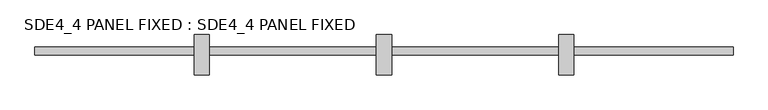
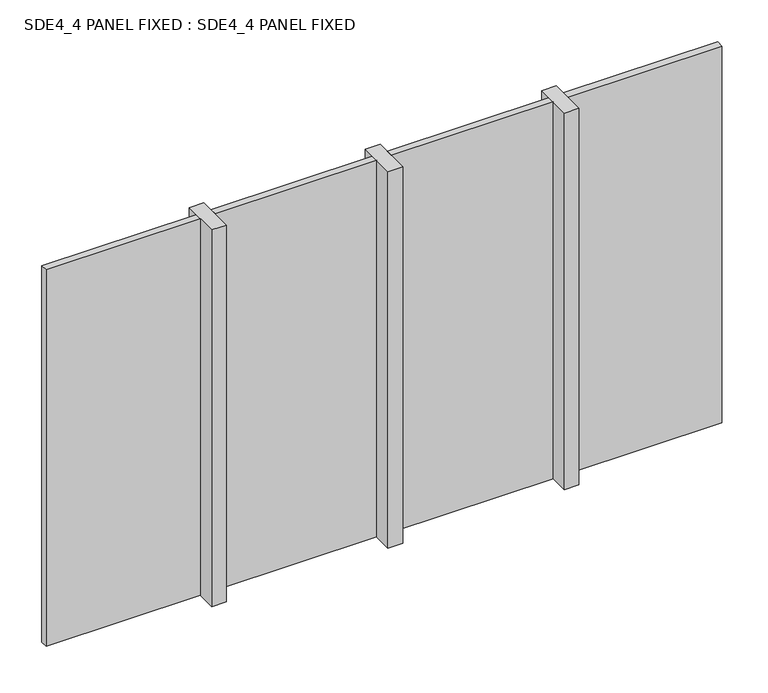
"""IFC4 building model written with IfcOpenShell, lengths in millimetres: plate geometry, SDE4_4 PANEL FIXED : SDE4_4 PANEL FIXED."""

from ifc_helpers import new_model, si_unit, origin, origin_with_axes, place, context, project, spatial, polyline, outline, extrude, source, transform, mapped, element, save


def sde4_4_panel_fixed_sde4_4_panel_fixed_547cd786(model_context):
    return source(origin(), model_context, "Body", "SweptSolid", [
        extrude(outline(polyline([(-1150.0, 132.5), (-1150.0, -132.5), (-1250.0, -132.5), (-1250.0, 132.5), (-1150.0, 132.5)])), origin_with_axes(), (0.0, 0.0, 1.0), 2710.0),
        extrude(outline(polyline([(50.0, 132.5), (50.0, -132.5), (-50.0, -132.5), (-50.0, 132.5), (50.0, 132.5)])), origin_with_axes(), (0.0, 0.0, 1.0), 2710.0),
        extrude(outline(polyline([(1250.0, 132.5), (1250.0, -132.5), (1150.0, -132.5), (1150.0, 132.5), (1250.0, 132.5)])), origin_with_axes(), (0.0, 0.0, 1.0), 2710.0),
        extrude(outline(polyline([(2299.0, 50.0), (2299.0, 0.0), (1250.0, 0.0), (1250.0, 50.0), (2299.0, 50.0)])), origin_with_axes(), (0.0, 0.0, 1.0), 2710.0),
        extrude(outline(polyline([(1150.0, 50.0), (1150.0, 0.0), (50.0, 0.0), (50.0, 50.0), (1150.0, 50.0)])), origin_with_axes(), (0.0, 0.0, 1.0), 2710.0),
        extrude(outline(polyline([(-50.0, 50.0), (-50.0, 0.0), (-1150.0, 0.0), (-1150.0, 50.0), (-50.0, 50.0)])), origin_with_axes(), (0.0, 0.0, 1.0), 2710.0),
        extrude(outline(polyline([(-1250.0, 50.0), (-1250.0, 0.0), (-2300.0, 0.0), (-2300.0, 50.0), (-1250.0, 50.0)])), origin_with_axes(), (0.0, 0.0, 1.0), 2710.0),
    ])


if __name__ == "__main__":
    model = new_model("IFC4")
    model_context = context("Model", 3, world=origin())
    ifc_project = project(units=[si_unit("LENGTHUNIT", "METRE", prefix="MILLI")], contexts=[model_context])
    site = spatial("IfcSite", under=ifc_project)
    building = spatial("IfcBuilding", under=site)
    placement = place(None, origin())
    sde4_4_panel_fixed_sde4_4_panel_fixed_shape = sde4_4_panel_fixed_sde4_4_panel_fixed_547cd786(model_context)
    element("IfcPlate", 1, ObjectType="SDE4_4 PANEL FIXED : SDE4_4 PANEL FIXED", at=placement, inside=building, context=model_context, shape_type="MappedRepresentation", body=[
        mapped(sde4_4_panel_fixed_sde4_4_panel_fixed_shape, transform((0.0, 0.0, 0.0), x_axis=(1.0, 0.0, 0.0), y_axis=(0.0, 1.0, 0.0), z_axis=(0.0, 0.0, 1.0))),
    ])
    save(model, "model.ifc")

# Revit data of these elements
# Type "SDE4_4 PANEL FIXED : SDE4_4 PANEL FIXED"
#   Type Mark = "CW-GLASS"
#   Analytic Construction = "<None>"
#   Glass = Glass
#   Frame = Aluminium
# Element 1 (IfcPlate, "SDE4_4 PANEL FIXED : SDE4_4 PANEL FIXED")
#   Materials on its faces: "Glass", "Aluminium"
# Materials
#   "Glass": class "Glass", colour RGB 0 128 192, transparency 0.9, Keynote = "L40", Cost = 0
#   "Aluminium": class "Unassigned", colour RGB 247 247 247, transparency 0, Cost = 0
